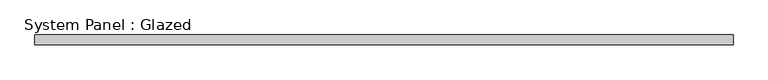
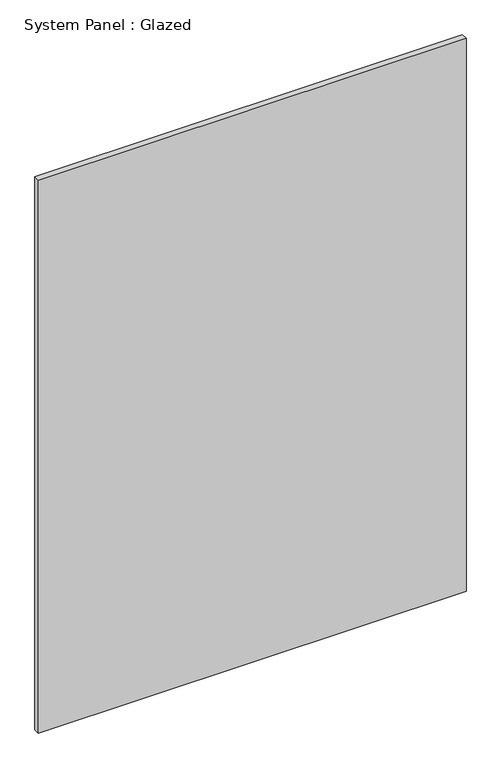
"""IFC4 building model written with IfcOpenShell, lengths in millimetres: plate geometry, System Panel : Glazed."""

import ifcopenshell
import ifcopenshell.guid

model = None  # the IFC model being written
_history = None  # IfcOwnerHistory: only IFC2X3 demands one
_inside = {}  # id of a spatial element -> (the spatial element, [elements in it])
_under = {}  # id of a project, library or spatial element -> (it, [spatial elements below it])
_declared = {}  # id of a project -> (the project, [libraries it declares])
_typed = {}  # id of a type object -> (the type object, [elements of that type])
_made_of = {}  # id of a material, layer set ... -> (it, [elements and type objects made of it])


def new_model(schema):
    """Start an empty IFC model of exactly this schema.

    Asked for "IFC4X3", IfcOpenShell would pick the latest addendum, in which some entities
    have other attributes; the version numbers below select the first issue.
    IFC2X3 requires an IfcOwnerHistory on every rooted entity: one is made here for all.
    """
    global model, _history
    if schema == "IFC4X3":
        model = ifcopenshell.file(schema_version=(4, 3, 0, 0))
    else:
        model = ifcopenshell.file(schema=schema)
    _inside.clear()
    _under.clear()
    _declared.clear()
    _typed.clear()
    _made_of.clear()
    _history = None
    if model.schema == "IFC2X3":
        org = make("IfcOrganization", Name="unknown")
        user = make(
            "IfcPersonAndOrganization",
            ThePerson=make("IfcPerson", FamilyName="unknown"),
            TheOrganization=org,
        )
        app = make(
            "IfcApplication",
            ApplicationDeveloper=org,
            Version="unknown",
            ApplicationFullName="unknown",
            ApplicationIdentifier="unknown",
        )
        _history = make(
            "IfcOwnerHistory",
            OwningUser=user,
            OwningApplication=app,
            ChangeAction="ADDED",
            CreationDate=0,
        )
    return model


def make(cls, **values):
    """One entity of the class cls with the attributes given. An attribute that is None is left unset."""
    return model.create_entity(
        cls, **{name: value for name, value in values.items() if value is not None}
    )


def rooted(cls, **values):
    """An entity with a GlobalId (a new one), such as an element, a storey or a relation."""
    return make(cls, GlobalId=ifcopenshell.guid.new(), OwnerHistory=_history, **values)


def si_unit(unit_type, name, prefix=None):
    """IfcSIUnit, for example si_unit("LENGTHUNIT", "METRE", prefix="MILLI")."""
    return make("IfcSIUnit", UnitType=unit_type, Prefix=prefix, Name=name)


def assignment(units):
    """IfcUnitAssignment: the units of a project."""
    return None if units is None else make("IfcUnitAssignment", Units=units)


def point(xyz):
    """IfcCartesianPoint."""
    return None if xyz is None else make("IfcCartesianPoint", Coordinates=xyz)


def direction(xyz):
    """IfcDirection."""
    return None if xyz is None else make("IfcDirection", DirectionRatios=xyz)


def frame(location, z_axis=None, x_axis=None):
    """IfcAxis2Placement3D, a coordinate frame: its origin and axes. An axis left out is left unset."""
    return make(
        "IfcAxis2Placement3D",
        Location=point(location),
        Axis=direction(z_axis),
        RefDirection=direction(x_axis),
    )


def origin():
    """The frame at (0, 0, 0) with its axes left unset."""
    return frame((0.0, 0.0, 0.0))


def origin_with_axes():
    """The frame at (0, 0, 0) with the z axis (0, 0, 1) and the x axis (1, 0, 0) written out."""
    return frame((0.0, 0.0, 0.0), z_axis=(0.0, 0.0, 1.0), x_axis=(1.0, 0.0, 0.0))


def place(relative_to, where):
    """IfcLocalPlacement: puts the frame where relative to a parent placement (None: the world)."""
    return make(
        "IfcLocalPlacement", PlacementRelTo=relative_to, RelativePlacement=where
    )


def context(
    kind, dimensions, precision=None, world=None, true_north=None, identifier=None
):
    """IfcGeometricRepresentationContext, for example the 3D "Model" context."""
    return make(
        "IfcGeometricRepresentationContext",
        ContextIdentifier=identifier,
        ContextType=kind,
        CoordinateSpaceDimension=dimensions,
        Precision=precision,
        WorldCoordinateSystem=world,
        TrueNorth=true_north,
    )


def project(units=None, contexts=None):
    """IfcProject with its units and contexts."""
    return rooted(
        "IfcProject",
        Name="project",
        RepresentationContexts=contexts,
        UnitsInContext=assignment(units),
    )


def spatial(cls, under=None, at=None, **own):
    """A site, building, storey or space (cls), placed at a placement, below another one or the project."""
    s = rooted(cls, ObjectPlacement=at, **own)
    if under is not None:
        _under.setdefault(under.id(), (under, []))[1].append(s)
    return s


def polyline(points):
    """IfcPolyline through the points."""
    return make("IfcPolyline", Points=[point(p) for p in points])


def outline(outer, holes=None, kind="AREA"):
    """IfcArbitraryClosedProfileDef: a profile drawn as a closed curve; with holes, ...WithVoids."""
    if holes is None:
        return make("IfcArbitraryClosedProfileDef", ProfileType=kind, OuterCurve=outer)
    return make(
        "IfcArbitraryProfileDefWithVoids",
        ProfileType=kind,
        OuterCurve=outer,
        InnerCurves=holes,
    )


def extrude(swept, where, along, depth):
    """IfcExtrudedAreaSolid: the profile swept, set in the frame where, extruded along a direction by depth."""
    return make(
        "IfcExtrudedAreaSolid",
        SweptArea=swept,
        Position=where,
        ExtrudedDirection=direction(along),
        Depth=depth,
    )


def shape(context_of_items, identifier, shape_type, items):
    """IfcShapeRepresentation: the items that make up one representation, for example the "Body"."""
    return make(
        "IfcShapeRepresentation",
        ContextOfItems=context_of_items,
        RepresentationIdentifier=identifier,
        RepresentationType=shape_type,
        Items=items,
    )


def source(mapping_origin, context_of_items, identifier, shape_type, items):
    """IfcRepresentationMap: a shape defined once, which mapped items show again and again."""
    return make(
        "IfcRepresentationMap",
        MappingOrigin=mapping_origin,
        MappedRepresentation=shape(context_of_items, identifier, shape_type, items),
    )


def transform(
    local_origin,
    x_axis=None,
    y_axis=None,
    z_axis=None,
    scale=None,
    scale2=None,
    scale3=None,
    uniform=True,
):
    """IfcCartesianTransformationOperator3D, or its non-uniform kind. x_axis, y_axis, z_axis: its Axis1, 2, 3."""
    if uniform:
        return make(
            "IfcCartesianTransformationOperator3D",
            Axis1=direction(x_axis),
            Axis2=direction(y_axis),
            LocalOrigin=point(local_origin),
            Scale=scale,
            Axis3=direction(z_axis),
        )
    return make(
        "IfcCartesianTransformationOperator3DnonUniform",
        Axis1=direction(x_axis),
        Axis2=direction(y_axis),
        LocalOrigin=point(local_origin),
        Scale=scale,
        Axis3=direction(z_axis),
        Scale2=scale2,
        Scale3=scale3,
    )


def mapped(mapping_source, mapping_target):
    """IfcMappedItem: shows the shape of a source again, moved by a transform."""
    return make(
        "IfcMappedItem", MappingSource=mapping_source, MappingTarget=mapping_target
    )


def made_of(thing, what):
    """Note that an element or type object is made of a material, layer set ...; save() writes the relation."""
    if what is not None:
        _made_of.setdefault(what.id(), (what, []))[1].append(thing)
    return thing


def element(
    cls,
    number,
    at=None,
    inside=None,
    cuts=None,
    type_object=None,
    material=None,
    context=None,
    identifier="Body",
    shape_type=None,
    held_by="IfcProductDefinitionShape",
    body=None,
    shapes=None,
    **own,
):
    """One element of the class cls, such as IfcWall. Its Tag is "e" and its number.

    at: its placement. inside: the storey or other place that contains it. cuts: it is an
    opening in that element (IfcRelVoidsElement). A single representation is given by context,
    identifier, shape_type and body (its items); several are given by shapes. held_by: the class
    of the entity that holds the representations. save() writes the other relations.
    """
    e = rooted(cls, Tag="e%d" % number, ObjectPlacement=at, **own)
    if body is not None:
        shapes = [shape(context, identifier, shape_type, body)]
    if shapes is not None:
        e.Representation = make(held_by, Representations=shapes)
    if inside is not None:
        _inside.setdefault(inside.id(), (inside, []))[1].append(e)
    if cuts is not None:
        rooted(
            "IfcRelVoidsElement", RelatingBuildingElement=cuts, RelatedOpeningElement=e
        )
    if type_object is not None:
        _typed.setdefault(type_object.id(), (type_object, []))[1].append(e)
    return made_of(e, material)


def aggregate(whole, parts):
    """IfcRelAggregates: a whole, such as a stair, and the parts it consists of."""
    return rooted("IfcRelAggregates", RelatingObject=whole, RelatedObjects=parts)


def save(model, path):
    """Write the relations noted so far, then the file.

    IfcRelAggregates (storeys below a building ...), IfcRelContainedInSpatialStructure (elements
    in a storey), IfcRelDefinesByType, IfcRelAssociatesMaterial and IfcRelDeclares: one each for
    every whole, place, type object, material and project.
    """
    for whole, parts in _under.values():
        aggregate(whole, parts)
    for where, things in _inside.values():
        rooted(
            "IfcRelContainedInSpatialStructure",
            RelatedElements=things,
            RelatingStructure=where,
        )
    for kind, things in _typed.values():
        rooted("IfcRelDefinesByType", RelatedObjects=things, RelatingType=kind)
    for what, things in _made_of.values():
        rooted("IfcRelAssociatesMaterial", RelatedObjects=things, RelatingMaterial=what)
    for by, libraries in _declared.values():
        rooted("IfcRelDeclares", RelatingContext=by, RelatedDefinitions=libraries)
    model.write(path)


def system_panel_glazed_bfc77baa(model_context):
    return source(origin(), model_context, "Body", "SweptSolid", [
        extrude(outline(polyline([(877.5000002, 24.5), (-877.5000002, 24.5), (-877.5000002, 49.5), (877.5000002, 49.5), (877.5000002, 24.5)])), origin_with_axes(), (0.0, 0.0, 1.0), 2400.0),
    ])


if __name__ == "__main__":
    model = new_model("IFC4")
    model_context = context("Model", 3, world=origin())
    ifc_project = project(units=[si_unit("LENGTHUNIT", "METRE", prefix="MILLI")], contexts=[model_context])
    site = spatial("IfcSite", under=ifc_project)
    building = spatial("IfcBuilding", under=site)
    placement = place(None, origin())
    system_panel_glazed_shape = system_panel_glazed_bfc77baa(model_context)
    element("IfcPlate", 1, ObjectType="System Panel : Glazed", at=placement, inside=building, context=model_context, shape_type="MappedRepresentation", body=[
        mapped(system_panel_glazed_shape, transform((0.0, 0.0, 0.0), x_axis=(1.0, 0.0, 0.0), y_axis=(0.0, 1.0, 0.0), z_axis=(0.0, 0.0, 1.0))),
    ])
    save(model, "model.ifc")

# Revit data of these elements
# Type "System Panel : Glazed"
#   Keynote = "H11"
#   Construction Type Id = "GSP4R"
#   Analytic Construction = "1/8 in Pilkington single glazing"
#   Visual Light Transmittance = 0.9
#   Solar Heat Gain Coefficient = 0.86
#   Heat Transfer Coefficient (U) = 6.7069 W/(m²·K)
#   Define Thermal Properties by = 1
# Element 1 (IfcPlate, "System Panel : Glazed")
#   Materials on its faces: "Glass"
# Materials
#   "Glass": class "Glass", colour RGB 0 128 192, transparency 0.9, Description = "Soda Lime Glass", Cost = 0
